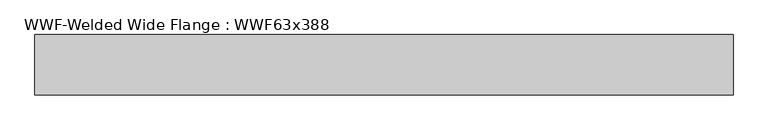
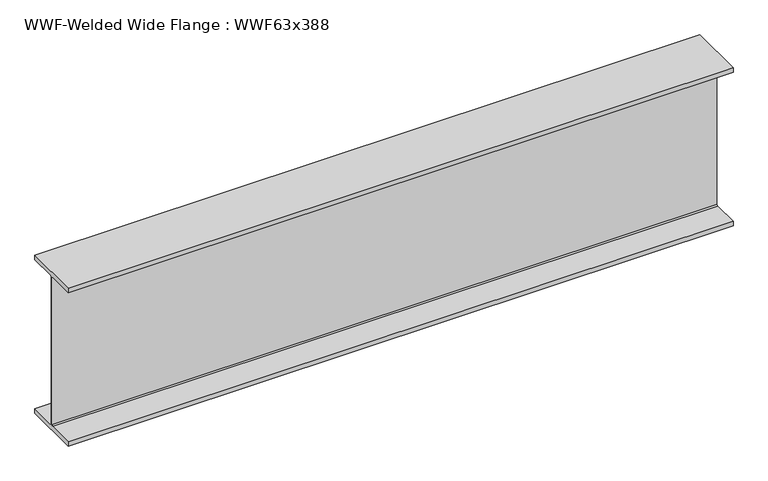
"""IFC4 building model written with IfcOpenShell, lengths in millimetres: beam geometry, WWF-Welded Wide Flange : WWF63x388."""

from ifc_helpers import new_model, si_unit, frame, origin, place, context, project, spatial, polyline, outline, extrude, source, transform, mapped, element, save


def wwf_welded_wide_flange_wwf63x388_cc5caaf4(model_context):
    return source(origin(), model_context, "Body", "SweptSolid", [
        extrude(outline(polyline([(274.955, -755.015), (274.955, -799.973), (-274.955, -799.973), (-274.955, -755.015), (-19.05, -755.015), (-8.001, -743.966), (-8.001, 743.966), (-19.05, 755.015), (-274.955, 755.015), (-274.955, 799.973), (274.955, 799.973), (274.955, 755.015), (19.05, 755.015), (8.001, 743.966), (8.001, -743.966), (19.05, -755.015), (274.955, -755.015)])), frame((-3184.569834, 0.0, 0.0), z_axis=(1.0, 0.0, 0.0), x_axis=(0.0, 1.0, 0.0)), (0.0, 0.0, 1.0), 6369.1344444),
    ])


if __name__ == "__main__":
    model = new_model("IFC4")
    model_context = context("Model", 3, world=origin())
    ifc_project = project(units=[si_unit("LENGTHUNIT", "METRE", prefix="MILLI")], contexts=[model_context])
    site = spatial("IfcSite", under=ifc_project)
    building = spatial("IfcBuilding", under=site)
    placement = place(None, origin())
    wwf_welded_wide_flange_wwf63x388_shape = wwf_welded_wide_flange_wwf63x388_cc5caaf4(model_context)
    element("IfcBeam", 1, ObjectType="WWF-Welded Wide Flange : WWF63x388", at=placement, inside=building, context=model_context, shape_type="MappedRepresentation", body=[
        mapped(wwf_welded_wide_flange_wwf63x388_shape, transform((0.0, 0.0, 0.0), x_axis=(1.0, 0.0, 0.0), y_axis=(0.0, 1.0, 0.0), z_axis=(0.0, 0.0, 1.0))),
    ])
    save(model, "model.ifc")

# Revit data of these elements
# Type "WWF-Welded Wide Flange : WWF63x388"
#   Assembly Code = "B10"
#   Nominal d = "12"
#   W = 388
#   Length [instance default] = 1524 mm
#   bf = 549.91 mm
#   d = 1599.946 mm
#   k = 19.05 mm
#   tf = 44.958 mm
#   tw = 16.002 mm
#   A = 0.0735482 m²
#   Structural Material [instance default] = Steel ASTM A572
# Element 1 (IfcBeam, "WWF-Welded Wide Flange : WWF63x388")
#   Structural Material = Metal - Steel 43-275
#   Materials on its faces: "Metal - Steel 43-275"
# Materials
#   "Steel ASTM A572": class "Metal", colour RGB 247 247 247, transparency 0, Description = "Structural steel, high strength low alloy, ASTM - A572 - 50", Cost = 0
#   "Metal - Steel 43-275": class "Metal", colour RGB 247 247 247, transparency 0, Cost = 0
